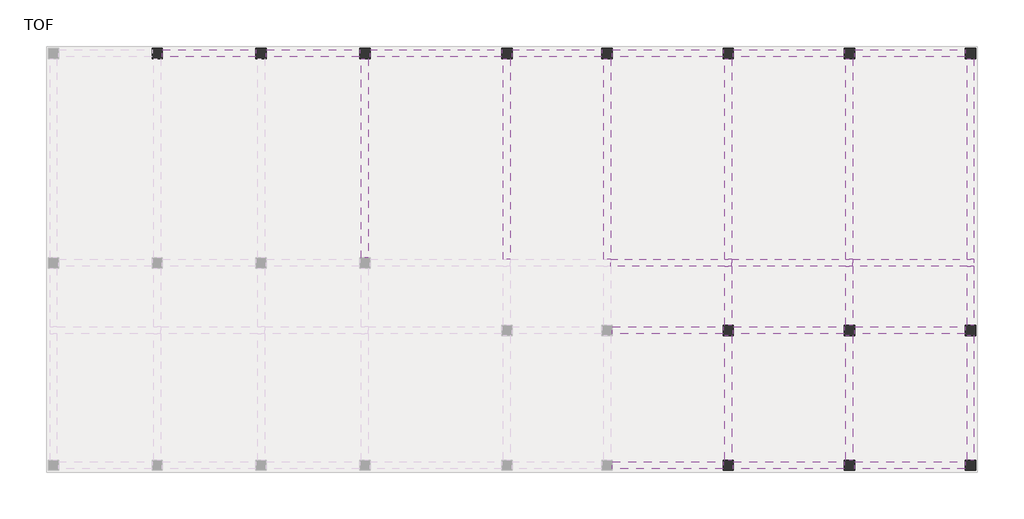
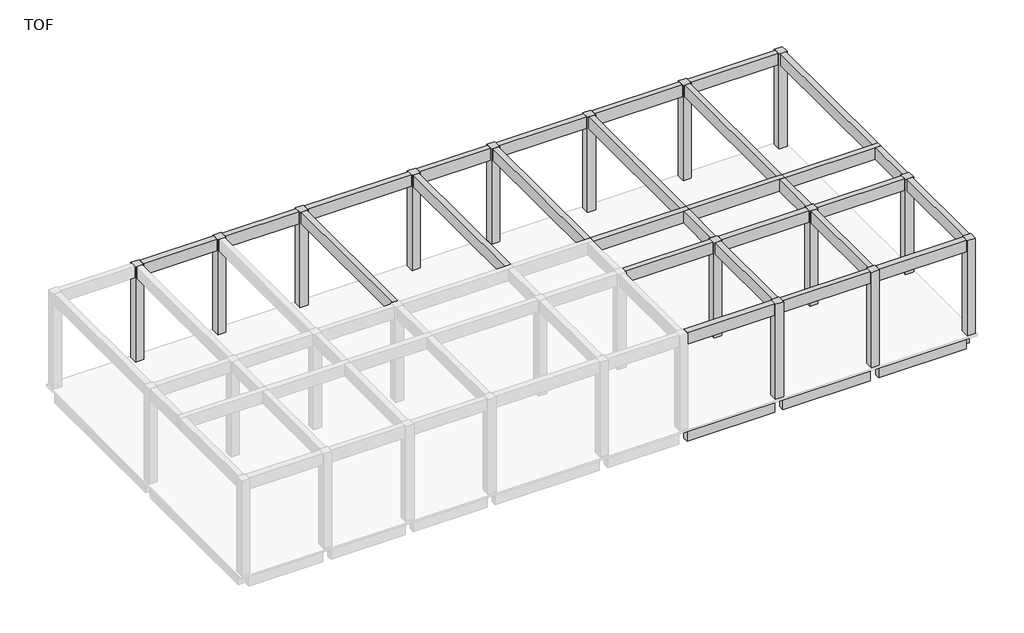
# One storey, part 2 of 2: 40 beams, 14 columns.
"""IFC4 building model written with IfcOpenShell, lengths in millimetres."""

from ifc_helpers import new_model, si_unit, frame, origin, place, context, project, spatial, polyline, outline, extrude, faceted_brep, element, save

model = new_model("IFC4")

# Units and contexts
model_context = context("Model", 3, world=origin())
ifc_project = project(units=[si_unit("LENGTHUNIT", "METRE", prefix="MILLI")], contexts=[model_context])

# Site, building, storey
site = spatial("IfcSite", under=ifc_project)
building = spatial("IfcBuilding", under=site)
storey = spatial("IfcBuildingStorey", under=building, Name="TOF", Elevation=150.0)

# Beams
placement = place(None, origin())
element("IfcBeam", 1, ObjectType="RC Beam_Rectangular : H_SB_ACB_B400xH900", at=placement, inside=storey, context=model_context, shape_type="SweptSolid", body=[
    extrude(outline(polyline([(52724.7, 24116.5208589), (53124.7, 24116.5208589), (53124.7, 18966.5208589), (52724.7, 18966.5208589), (52724.7, 24116.5208589)])), frame((0.0, 0.0, -900.0), z_axis=(0.0, 0.0, 1.0), x_axis=(1.0, 0.0, 0.0)), (0.0, 0.0, 1.0), 900.0),
    extrude(outline(polyline([(53124.7, 8716.5208589), (52724.7, 8716.5208589), (52724.7, 18366.5208589), (53124.7, 18366.5208589), (53124.7, 8716.5208589)])), frame((0.0, 0.0, -900.0), z_axis=(0.0, 0.0, 1.0), x_axis=(1.0, 0.0, 0.0)), (0.0, 0.0, 1.0), 900.0),
])
element("IfcBeam", 2, ObjectType="RC Beam_Rectangular : H_SB_ACB_B400xH900", at=placement, inside=storey, context=model_context, shape_type="SweptSolid", body=[
    extrude(outline(polyline([(52724.7, 8116.5208589), (53124.7, 8116.5208589), (53124.7, 916.5208589), (52724.7, 916.5208589), (52724.7, 8116.5208589)])), frame((0.0, 0.0, -900.0), z_axis=(0.0, 0.0, 1.0), x_axis=(1.0, 0.0, 0.0)), (0.0, 0.0, 1.0), 900.0),
])
element("IfcBeam", 3, ObjectType="RC Beam_Rectangular : H_SB_ACB_B400xH900", at=placement, inside=storey, context=model_context, shape_type="SweptSolid", body=[
    extrude(outline(polyline([(6224.7, 24216.5208589), (6224.7, 24616.5208589), (11624.7, 24616.5208589), (11624.7, 24216.5208589), (6224.7, 24216.5208589)])), frame((0.0, 0.0, -900.0), z_axis=(0.0, 0.0, 1.0), x_axis=(1.0, 0.0, 0.0)), (0.0, 0.0, 1.0), 900.0),
])
element("IfcBeam", 4, ObjectType="RC Beam_Rectangular : H_SB_ACB_B400xH900", at=placement, inside=storey, context=model_context, shape_type="SweptSolid", body=[
    extrude(outline(polyline([(12224.7, 24216.5208589), (12224.7, 24616.5208589), (17624.7, 24616.5208589), (17624.7, 24216.5208589), (12224.7, 24216.5208589)])), frame((0.0, 0.0, -900.0), z_axis=(0.0, 0.0, 1.0), x_axis=(1.0, 0.0, 0.0)), (0.0, 0.0, 1.0), 900.0),
])
element("IfcBeam", 5, ObjectType="RC Beam_Rectangular : H_SB_ACB_B400xH900", at=placement, inside=storey, context=model_context, shape_type="SweptSolid", body=[
    extrude(outline(polyline([(18224.7, 24216.5208589), (18224.7, 24616.5208589), (25824.7, 24616.5208589), (25824.7, 24216.5208589), (18224.7, 24216.5208589)])), frame((0.0, 0.0, -900.0), z_axis=(0.0, 0.0, 1.0), x_axis=(1.0, 0.0, 0.0)), (0.0, 0.0, 1.0), 900.0),
])
element("IfcBeam", 6, ObjectType="RC Beam_Rectangular : H_SB_ACB_B400xH900", at=placement, inside=storey, context=model_context, shape_type="SweptSolid", body=[
    extrude(outline(polyline([(26424.7, 24216.5208589), (26424.7, 24616.5208589), (31624.7, 24616.5208589), (31624.7, 24216.5208589), (26424.7, 24216.5208589)])), frame((0.0, 0.0, -900.0), z_axis=(0.0, 0.0, 1.0), x_axis=(1.0, 0.0, 0.0)), (0.0, 0.0, 1.0), 900.0),
])
element("IfcBeam", 7, ObjectType="RC Beam_Rectangular : H_SB_ACB_B400xH900", at=placement, inside=storey, context=model_context, shape_type="SweptSolid", body=[
    extrude(outline(polyline([(32224.7, 24216.5208589), (32224.7, 24616.5208589), (38624.7, 24616.5208589), (38624.7, 24216.5208589), (32224.7, 24216.5208589)])), frame((0.0, 0.0, -900.0), z_axis=(0.0, 0.0, 1.0), x_axis=(1.0, 0.0, 0.0)), (0.0, 0.0, 1.0), 900.0),
])
element("IfcBeam", 8, ObjectType="RC Beam_Rectangular : H_SB_ACB_B400xH900", at=placement, inside=storey, context=model_context, shape_type="SweptSolid", body=[
    extrude(outline(polyline([(39224.7, 24216.5208589), (39224.7, 24616.5208589), (45624.7, 24616.5208589), (45624.7, 24216.5208589), (39224.7, 24216.5208589)])), frame((0.0, 0.0, -900.0), z_axis=(0.0, 0.0, 1.0), x_axis=(1.0, 0.0, 0.0)), (0.0, 0.0, 1.0), 900.0),
])
element("IfcBeam", 9, ObjectType="RC Beam_Rectangular : H_SB_ACB_B400xH900", at=placement, inside=storey, context=model_context, shape_type="SweptSolid", body=[
    extrude(outline(polyline([(46224.7, 24216.5208589), (46224.7, 24616.5208589), (52624.7, 24616.5208589), (52624.7, 24216.5208589), (46224.7, 24216.5208589)])), frame((0.0, 0.0, -900.0), z_axis=(0.0, 0.0, 1.0), x_axis=(1.0, 0.0, 0.0)), (0.0, 0.0, 1.0), 900.0),
])
element("IfcBeam", 10, ObjectType="RC Beam_Rectangular : H_SB_ACB_B400xH900", at=placement, inside=storey, context=model_context, shape_type="SweptSolid", body=[
    extrude(outline(polyline([(32224.7, 416.5208589), (32224.7, 816.5208589), (38624.7, 816.5208589), (38624.7, 416.5208589), (32224.7, 416.5208589)])), frame((0.0, 0.0, -900.0), z_axis=(0.0, 0.0, 1.0), x_axis=(1.0, 0.0, 0.0)), (0.0, 0.0, 1.0), 900.0),
])
element("IfcBeam", 11, ObjectType="RC Beam_Rectangular : H_SB_ACB_B400xH900", at=placement, inside=storey, context=model_context, shape_type="SweptSolid", body=[
    extrude(outline(polyline([(39224.7, 416.5208589), (39224.7, 816.5208589), (45624.7, 816.5208589), (45624.7, 416.5208589), (39224.7, 416.5208589)])), frame((0.0, 0.0, -900.0), z_axis=(0.0, 0.0, 1.0), x_axis=(1.0, 0.0, 0.0)), (0.0, 0.0, 1.0), 900.0),
])
element("IfcBeam", 12, ObjectType="RC Beam_Rectangular : H_SB_ACB_B400xH900", at=placement, inside=storey, context=model_context, shape_type="SweptSolid", body=[
    extrude(outline(polyline([(46224.7, 416.5208589), (46224.7, 816.5208589), (52624.7, 816.5208589), (52624.7, 416.5208589), (46224.7, 416.5208589)])), frame((0.0, 0.0, -900.0), z_axis=(0.0, 0.0, 1.0), x_axis=(1.0, 0.0, 0.0)), (0.0, 0.0, 1.0), 900.0),
])
element("IfcBeam", 13, ObjectType="RC Beam_Rectangular : H_SB_ACB_B400xH900", at=placement, inside=storey, context=model_context, shape_type="Brep", body=[
    faceted_brep([(39124.7, 12116.5208589, 7500.0), (39124.7, 12516.5208589, 7500.0), (38724.7, 12516.5208589, 7500.0), (32124.7, 12516.5208589, 7500.0), (32124.7, 12116.5208589, 7500.0), (38724.7, 12116.5208589, 7500.0), (39124.7, 12116.5208589, 6600.0), (32124.7, 12116.5208589, 6600.0), (38724.7, 12116.5208589, 6600.0), (39124.7, 12516.5208589, 6600.0), (32124.7, 12516.5208589, 6600.0), (38724.7, 12516.5208589, 6600.0)], [[[0, 1, 2, 3, 4, 5]], [[6, 0, 5, 4, 7, 8]], [[9, 6, 8, 7, 10, 11]], [[1, 9, 11, 10, 3, 2]], [[1, 0, 6, 9]], [[4, 3, 10, 7]]]),
])
element("IfcBeam", 14, ObjectType="RC Beam_Rectangular : H_SB_ACB_B400xH900", at=placement, inside=storey, context=model_context, shape_type="Brep", body=[
    faceted_brep([(46124.7, 12116.5208589, 7500.0), (46124.7, 12516.5208589, 7500.0), (45724.7, 12516.5208589, 7500.0), (39124.7, 12516.5208589, 7500.0), (39124.7, 12116.5208589, 7500.0), (45724.7, 12116.5208589, 7500.0), (46124.7, 12116.5208589, 6600.0), (39124.7, 12116.5208589, 6600.0), (45724.7, 12116.5208589, 6600.0), (46124.7, 12516.5208589, 6600.0), (39124.7, 12516.5208589, 6600.0), (45724.7, 12516.5208589, 6600.0)], [[[0, 1, 2, 3, 4, 5]], [[6, 0, 5, 4, 7, 8]], [[9, 6, 8, 7, 10, 11]], [[1, 9, 11, 10, 3, 2]], [[1, 0, 6, 9]], [[4, 3, 10, 7]]]),
])
element("IfcBeam", 15, ObjectType="RC Beam_Rectangular : H_SB_ACB_B400xH900", at=placement, inside=storey, context=model_context, shape_type="Brep", body=[
    faceted_brep([(53124.7, 12116.5208589, 7500.0), (53124.7, 12516.5208589, 7500.0), (52724.7, 12516.5208589, 7500.0), (46124.7, 12516.5208589, 7500.0), (46124.7, 12116.5208589, 7500.0), (52724.7, 12116.5208589, 7500.0), (53124.7, 12116.5208589, 6600.0), (46124.7, 12116.5208589, 6600.0), (52724.7, 12116.5208589, 6600.0), (53124.7, 12516.5208589, 6600.0), (46124.7, 12516.5208589, 6600.0), (52724.7, 12516.5208589, 6600.0)], [[[0, 1, 2, 3, 4, 5]], [[6, 0, 5, 4, 7, 8]], [[9, 6, 8, 7, 10, 11]], [[1, 9, 11, 10, 3, 2]], [[1, 0, 6, 9]], [[4, 3, 10, 7]]]),
])
element("IfcBeam", 16, ObjectType="RC Beam_Rectangular : H_SB_ACB_B400xH900", at=placement, inside=storey, context=model_context, shape_type="SweptSolid", body=[
    extrude(outline(polyline([(6224.7, 24216.5208589), (6224.7, 24616.5208589), (11624.7, 24616.5208589), (11624.7, 24216.5208589), (6224.7, 24216.5208589)])), frame((0.0, 0.0, 6600.0), z_axis=(0.0, 0.0, 1.0), x_axis=(1.0, 0.0, 0.0)), (0.0, 0.0, 1.0), 900.0),
])
element("IfcBeam", 17, ObjectType="RC Beam_Rectangular : H_SB_ACB_B400xH900", at=placement, inside=storey, context=model_context, shape_type="SweptSolid", body=[
    extrude(outline(polyline([(12224.7, 24216.5208589), (12224.7, 24616.5208589), (17624.7, 24616.5208589), (17624.7, 24216.5208589), (12224.7, 24216.5208589)])), frame((0.0, 0.0, 6600.0), z_axis=(0.0, 0.0, 1.0), x_axis=(1.0, 0.0, 0.0)), (0.0, 0.0, 1.0), 900.0),
])
element("IfcBeam", 18, ObjectType="RC Beam_Rectangular : H_SB_ACB_B400xH900", at=placement, inside=storey, context=model_context, shape_type="SweptSolid", body=[
    extrude(outline(polyline([(18224.7, 24216.5208589), (18224.7, 24616.5208589), (25824.7, 24616.5208589), (25824.7, 24216.5208589), (18224.7, 24216.5208589)])), frame((0.0, 0.0, 6600.0), z_axis=(0.0, 0.0, 1.0), x_axis=(1.0, 0.0, 0.0)), (0.0, 0.0, 1.0), 900.0),
])
element("IfcBeam", 19, ObjectType="RC Beam_Rectangular : H_SB_ACB_B400xH900", at=placement, inside=storey, context=model_context, shape_type="SweptSolid", body=[
    extrude(outline(polyline([(26424.7, 24216.5208589), (26424.7, 24616.5208589), (31624.7, 24616.5208589), (31624.7, 24216.5208589), (26424.7, 24216.5208589)])), frame((0.0, 0.0, 6600.0), z_axis=(0.0, 0.0, 1.0), x_axis=(1.0, 0.0, 0.0)), (0.0, 0.0, 1.0), 900.0),
])
element("IfcBeam", 20, ObjectType="RC Beam_Rectangular : H_SB_ACB_B400xH900", at=placement, inside=storey, context=model_context, shape_type="SweptSolid", body=[
    extrude(outline(polyline([(32224.7, 24216.5208589), (32224.7, 24616.5208589), (38624.7, 24616.5208589), (38624.7, 24216.5208589), (32224.7, 24216.5208589)])), frame((0.0, 0.0, 6600.0), z_axis=(0.0, 0.0, 1.0), x_axis=(1.0, 0.0, 0.0)), (0.0, 0.0, 1.0), 900.0),
])
element("IfcBeam", 21, ObjectType="RC Beam_Rectangular : H_SB_ACB_B400xH900", at=placement, inside=storey, context=model_context, shape_type="SweptSolid", body=[
    extrude(outline(polyline([(39224.7, 24216.5208589), (39224.7, 24616.5208589), (45624.7, 24616.5208589), (45624.7, 24216.5208589), (39224.7, 24216.5208589)])), frame((0.0, 0.0, 6600.0), z_axis=(0.0, 0.0, 1.0), x_axis=(1.0, 0.0, 0.0)), (0.0, 0.0, 1.0), 900.0),
])
element("IfcBeam", 22, ObjectType="RC Beam_Rectangular : H_SB_ACB_B400xH900", at=placement, inside=storey, context=model_context, shape_type="SweptSolid", body=[
    extrude(outline(polyline([(46224.7, 24216.5208589), (46224.7, 24616.5208589), (52624.7, 24616.5208589), (52624.7, 24216.5208589), (46224.7, 24216.5208589)])), frame((0.0, 0.0, 6600.0), z_axis=(0.0, 0.0, 1.0), x_axis=(1.0, 0.0, 0.0)), (0.0, 0.0, 1.0), 900.0),
])
element("IfcBeam", 23, ObjectType="RC Beam_Rectangular : H_SB_ACB_B400xH900", at=placement, inside=storey, context=model_context, shape_type="SweptSolid", body=[
    extrude(outline(polyline([(32224.7, 8216.5208589), (32224.7, 8616.5208589), (38624.7, 8616.5208589), (38624.7, 8216.5208589), (32224.7, 8216.5208589)])), frame((0.0, 0.0, 6600.0), z_axis=(0.0, 0.0, 1.0), x_axis=(1.0, 0.0, 0.0)), (0.0, 0.0, 1.0), 900.0),
])
element("IfcBeam", 24, ObjectType="RC Beam_Rectangular : H_SB_ACB_B400xH900", at=placement, inside=storey, context=model_context, shape_type="SweptSolid", body=[
    extrude(outline(polyline([(39224.7, 8216.5208589), (39224.7, 8616.5208589), (45624.7, 8616.5208589), (45624.7, 8216.5208589), (39224.7, 8216.5208589)])), frame((0.0, 0.0, 6600.0), z_axis=(0.0, 0.0, 1.0), x_axis=(1.0, 0.0, 0.0)), (0.0, 0.0, 1.0), 900.0),
])
element("IfcBeam", 25, ObjectType="RC Beam_Rectangular : H_SB_ACB_B400xH900", at=placement, inside=storey, context=model_context, shape_type="SweptSolid", body=[
    extrude(outline(polyline([(46224.7, 8216.5208589), (46224.7, 8616.5208589), (52624.7, 8616.5208589), (52624.7, 8216.5208589), (46224.7, 8216.5208589)])), frame((0.0, 0.0, 6600.0), z_axis=(0.0, 0.0, 1.0), x_axis=(1.0, 0.0, 0.0)), (0.0, 0.0, 1.0), 900.0),
])
element("IfcBeam", 26, ObjectType="RC Beam_Rectangular : H_SB_ACB_B400xH900", at=placement, inside=storey, context=model_context, shape_type="SweptSolid", body=[
    extrude(outline(polyline([(32224.7, 416.5208589), (32224.7, 816.5208589), (38624.7, 816.5208589), (38624.7, 416.5208589), (32224.7, 416.5208589)])), frame((0.0, 0.0, 6600.0), z_axis=(0.0, 0.0, 1.0), x_axis=(1.0, 0.0, 0.0)), (0.0, 0.0, 1.0), 900.0),
])
element("IfcBeam", 27, ObjectType="RC Beam_Rectangular : H_SB_ACB_B400xH900", at=placement, inside=storey, context=model_context, shape_type="SweptSolid", body=[
    extrude(outline(polyline([(39224.7, 416.5208589), (39224.7, 816.5208589), (45624.7, 816.5208589), (45624.7, 416.5208589), (39224.7, 416.5208589)])), frame((0.0, 0.0, 6600.0), z_axis=(0.0, 0.0, 1.0), x_axis=(1.0, 0.0, 0.0)), (0.0, 0.0, 1.0), 900.0),
])
element("IfcBeam", 28, ObjectType="RC Beam_Rectangular : H_SB_ACB_B400xH900", at=placement, inside=storey, context=model_context, shape_type="SweptSolid", body=[
    extrude(outline(polyline([(46224.7, 416.5208589), (46224.7, 816.5208589), (52624.7, 816.5208589), (52624.7, 416.5208589), (46224.7, 416.5208589)])), frame((0.0, 0.0, 6600.0), z_axis=(0.0, 0.0, 1.0), x_axis=(1.0, 0.0, 0.0)), (0.0, 0.0, 1.0), 900.0),
])
element("IfcBeam", 29, ObjectType="RC Beam_Rectangular : H_SB_ACB_B400xH900", at=placement, inside=storey, context=model_context, shape_type="SweptSolid", body=[
    extrude(outline(polyline([(18124.7, 12616.5208589), (17724.7, 12616.5208589), (17724.7, 24116.5208589), (18124.7, 24116.5208589), (18124.7, 12616.5208589)])), frame((0.0, 0.0, 6600.0), z_axis=(0.0, 0.0, 1.0), x_axis=(1.0, 0.0, 0.0)), (0.0, 0.0, 1.0), 900.0),
])
element("IfcBeam", 30, ObjectType="RC Beam_Rectangular : H_SB_ACB_B400xH900", at=placement, inside=storey, context=model_context, shape_type="SweptSolid", body=[
    extrude(outline(polyline([(26324.7, 12516.5208589), (25924.7, 12516.5208589), (25924.7, 24116.5208589), (26324.7, 24116.5208589), (26324.7, 12516.5208589)])), frame((0.0, 0.0, 6600.0), z_axis=(0.0, 0.0, 1.0), x_axis=(1.0, 0.0, 0.0)), (0.0, 0.0, 1.0), 900.0),
])
element("IfcBeam", 31, ObjectType="RC Beam_Rectangular : H_SB_ACB_B400xH900", at=placement, inside=storey, context=model_context, shape_type="SweptSolid", body=[
    extrude(outline(polyline([(32124.7, 12516.5208589), (31724.7, 12516.5208589), (31724.7, 24116.5208589), (32124.7, 24116.5208589), (32124.7, 12516.5208589)])), frame((0.0, 0.0, 6600.0), z_axis=(0.0, 0.0, 1.0), x_axis=(1.0, 0.0, 0.0)), (0.0, 0.0, 1.0), 900.0),
])
element("IfcBeam", 32, ObjectType="RC Beam_Rectangular : H_SB_ACB_B400xH900", at=placement, inside=storey, context=model_context, shape_type="SweptSolid", body=[
    extrude(outline(polyline([(38724.7, 8116.5208589), (39124.7, 8116.5208589), (39124.7, 916.5208589), (38724.7, 916.5208589), (38724.7, 8116.5208589)])), frame((0.0, 0.0, 6600.0), z_axis=(0.0, 0.0, 1.0), x_axis=(1.0, 0.0, 0.0)), (0.0, 0.0, 1.0), 900.0),
])
element("IfcBeam", 33, ObjectType="RC Beam_Rectangular : H_SB_ACB_B400xH900", at=placement, inside=storey, context=model_context, shape_type="SweptSolid", body=[
    extrude(outline(polyline([(38724.7, 12116.5208589), (39124.7, 12116.5208589), (39124.7, 8716.5208589), (38724.7, 8716.5208589), (38724.7, 12116.5208589)])), frame((0.0, 0.0, 6600.0), z_axis=(0.0, 0.0, 1.0), x_axis=(1.0, 0.0, 0.0)), (0.0, 0.0, 1.0), 900.0),
])
element("IfcBeam", 34, ObjectType="RC Beam_Rectangular : H_SB_ACB_B400xH900", at=placement, inside=storey, context=model_context, shape_type="SweptSolid", body=[
    extrude(outline(polyline([(39124.7, 12516.5208589), (38724.7, 12516.5208589), (38724.7, 24116.5208589), (39124.7, 24116.5208589), (39124.7, 12516.5208589)])), frame((0.0, 0.0, 6600.0), z_axis=(0.0, 0.0, 1.0), x_axis=(1.0, 0.0, 0.0)), (0.0, 0.0, 1.0), 900.0),
])
element("IfcBeam", 35, ObjectType="RC Beam_Rectangular : H_SB_ACB_B400xH900", at=placement, inside=storey, context=model_context, shape_type="SweptSolid", body=[
    extrude(outline(polyline([(45724.7, 8116.5208589), (46124.7, 8116.5208589), (46124.7, 916.5208589), (45724.7, 916.5208589), (45724.7, 8116.5208589)])), frame((0.0, 0.0, 6600.0), z_axis=(0.0, 0.0, 1.0), x_axis=(1.0, 0.0, 0.0)), (0.0, 0.0, 1.0), 900.0),
])
element("IfcBeam", 36, ObjectType="RC Beam_Rectangular : H_SB_ACB_B400xH900", at=placement, inside=storey, context=model_context, shape_type="SweptSolid", body=[
    extrude(outline(polyline([(45724.7, 12116.5208589), (46124.7, 12116.5208589), (46124.7, 8716.5208589), (45724.7, 8716.5208589), (45724.7, 12116.5208589)])), frame((0.0, 0.0, 6600.0), z_axis=(0.0, 0.0, 1.0), x_axis=(1.0, 0.0, 0.0)), (0.0, 0.0, 1.0), 900.0),
])
element("IfcBeam", 37, ObjectType="RC Beam_Rectangular : H_SB_ACB_B400xH900", at=placement, inside=storey, context=model_context, shape_type="SweptSolid", body=[
    extrude(outline(polyline([(46124.7, 12516.5208589), (45724.7, 12516.5208589), (45724.7, 24116.5208589), (46124.7, 24116.5208589), (46124.7, 12516.5208589)])), frame((0.0, 0.0, 6600.0), z_axis=(0.0, 0.0, 1.0), x_axis=(1.0, 0.0, 0.0)), (0.0, 0.0, 1.0), 900.0),
])
element("IfcBeam", 38, ObjectType="RC Beam_Rectangular : H_SB_ACB_B400xH900", at=placement, inside=storey, context=model_context, shape_type="SweptSolid", body=[
    extrude(outline(polyline([(52724.7, 8116.5208589), (53124.7, 8116.5208589), (53124.7, 916.5208589), (52724.7, 916.5208589), (52724.7, 8116.5208589)])), frame((0.0, 0.0, 6600.0), z_axis=(0.0, 0.0, 1.0), x_axis=(1.0, 0.0, 0.0)), (0.0, 0.0, 1.0), 900.0),
])
element("IfcBeam", 39, ObjectType="RC Beam_Rectangular : H_SB_ACB_B400xH900", at=placement, inside=storey, context=model_context, shape_type="SweptSolid", body=[
    extrude(outline(polyline([(52724.7, 12116.5208589), (53124.7, 12116.5208589), (53124.7, 8716.5208589), (52724.7, 8716.5208589), (52724.7, 12116.5208589)])), frame((0.0, 0.0, 6600.0), z_axis=(0.0, 0.0, 1.0), x_axis=(1.0, 0.0, 0.0)), (0.0, 0.0, 1.0), 900.0),
])
element("IfcBeam", 40, ObjectType="RC Beam_Rectangular : H_SB_ACB_B400xH900", at=placement, inside=storey, context=model_context, shape_type="SweptSolid", body=[
    extrude(outline(polyline([(52724.7, 24116.5208589), (53124.7, 24116.5208589), (53124.7, 12516.5208589), (52724.7, 12516.5208589), (52724.7, 24116.5208589)])), frame((0.0, 0.0, 6600.0), z_axis=(0.0, 0.0, 1.0), x_axis=(1.0, 0.0, 0.0)), (0.0, 0.0, 1.0), 900.0),
])

# Columns
element("IfcColumn", 41, ObjectType="RC_Column_Rectangular : H_SC_ACC_W600xL600", at=placement, inside=storey, context=model_context, shape_type="Brep", body=[
    faceted_brep([(6224.7, 24716.5208589, 7500.0), (6224.7, 24616.5208589, 7500.0), (6224.7, 24216.5208589, 7500.0), (6224.7, 24116.5208589, 7500.0), (6224.7, 24116.5208589, 150.0), (6224.7, 24716.5208589, 150.0), (6124.7, 24116.5208589, 7500.0), (5724.7, 24116.5208589, 7500.0), (5624.7, 24116.5208589, 7500.0), (5624.7, 24116.5208589, 150.0), (5624.7, 24216.5208589, 7500.0), (5624.7, 24616.5208589, 7500.0), (5624.7, 24716.5208589, 7500.0), (5624.7, 24716.5208589, 150.0)], [[[0, 1, 2, 3, 4, 5]], [[3, 6, 7, 8, 9, 4]], [[8, 10, 11, 12, 13, 9]], [[12, 0, 5, 13]], [[3, 2, 1, 0, 12, 11, 10, 8, 7, 6]], [[5, 4, 9, 13]]]),
])
element("IfcColumn", 42, ObjectType="RC_Column_Rectangular : H_SC_ACC_W600xL600", at=placement, inside=storey, context=model_context, shape_type="Brep", body=[
    faceted_brep([(12224.7, 24716.5208589, 7500.0), (12224.7, 24616.5208589, 7500.0), (12224.7, 24216.5208589, 7500.0), (12224.7, 24116.5208589, 7500.0), (12224.7, 24116.5208589, 150.0), (12224.7, 24716.5208589, 150.0), (12124.7, 24116.5208589, 7500.0), (11724.7, 24116.5208589, 7500.0), (11624.7, 24116.5208589, 7500.0), (11624.7, 24116.5208589, 150.0), (11624.7, 24216.5208589, 7500.0), (11624.7, 24616.5208589, 7500.0), (11624.7, 24716.5208589, 7500.0), (11624.7, 24716.5208589, 150.0)], [[[0, 1, 2, 3, 4, 5]], [[3, 6, 7, 8, 9, 4]], [[8, 10, 11, 12, 13, 9]], [[12, 0, 5, 13]], [[3, 2, 1, 0, 12, 11, 10, 8, 7, 6]], [[5, 4, 9, 13]]]),
])
element("IfcColumn", 43, ObjectType="RC_Column_Rectangular : H_SC_ACC_W600xL600", at=placement, inside=storey, context=model_context, shape_type="Brep", body=[
    faceted_brep([(18224.7, 24716.5208589, 7500.0), (18224.7, 24616.5208589, 7500.0), (18224.7, 24216.5208589, 7500.0), (18224.7, 24116.5208589, 7500.0), (18224.7, 24116.5208589, 150.0), (18224.7, 24716.5208589, 150.0), (18124.7, 24116.5208589, 7500.0), (17724.7, 24116.5208589, 7500.0), (17624.7, 24116.5208589, 7500.0), (17624.7, 24116.5208589, 150.0), (17624.7, 24216.5208589, 7500.0), (17624.7, 24616.5208589, 7500.0), (17624.7, 24716.5208589, 7500.0), (17624.7, 24716.5208589, 150.0)], [[[0, 1, 2, 3, 4, 5]], [[3, 6, 7, 8, 9, 4]], [[8, 10, 11, 12, 13, 9]], [[12, 0, 5, 13]], [[3, 2, 1, 0, 12, 11, 10, 8, 7, 6]], [[5, 4, 9, 13]]]),
])
element("IfcColumn", 44, ObjectType="RC_Column_Rectangular : H_SC_ACC_W600xL600", at=placement, inside=storey, context=model_context, shape_type="Brep", body=[
    faceted_brep([(26424.7, 24716.5208589, 7500.0), (26424.7, 24616.5208589, 7500.0), (26424.7, 24216.5208589, 7500.0), (26424.7, 24116.5208589, 7500.0), (26424.7, 24116.5208589, 150.0), (26424.7, 24716.5208589, 150.0), (26324.7, 24116.5208589, 7500.0), (25924.7, 24116.5208589, 7500.0), (25824.7, 24116.5208589, 7500.0), (25824.7, 24116.5208589, 150.0), (25824.7, 24216.5208589, 7500.0), (25824.7, 24616.5208589, 7500.0), (25824.7, 24716.5208589, 7500.0), (25824.7, 24716.5208589, 150.0)], [[[0, 1, 2, 3, 4, 5]], [[3, 6, 7, 8, 9, 4]], [[8, 10, 11, 12, 13, 9]], [[12, 0, 5, 13]], [[3, 2, 1, 0, 12, 11, 10, 8, 7, 6]], [[5, 4, 9, 13]]]),
])
element("IfcColumn", 45, ObjectType="RC_Column_Rectangular : H_SC_ACC_W600xL600", at=placement, inside=storey, context=model_context, shape_type="Brep", body=[
    faceted_brep([(32224.7, 24716.5208589, 7500.0), (32224.7, 24616.5208589, 7500.0), (32224.7, 24216.5208589, 7500.0), (32224.7, 24116.5208589, 7500.0), (32224.7, 24116.5208589, 150.0), (32224.7, 24716.5208589, 150.0), (32124.7, 24116.5208589, 7500.0), (31724.7, 24116.5208589, 7500.0), (31624.7, 24116.5208589, 7500.0), (31624.7, 24116.5208589, 150.0), (31624.7, 24216.5208589, 7500.0), (31624.7, 24616.5208589, 7500.0), (31624.7, 24716.5208589, 7500.0), (31624.7, 24716.5208589, 150.0)], [[[0, 1, 2, 3, 4, 5]], [[3, 6, 7, 8, 9, 4]], [[8, 10, 11, 12, 13, 9]], [[12, 0, 5, 13]], [[3, 2, 1, 0, 12, 11, 10, 8, 7, 6]], [[5, 4, 9, 13]]]),
])
element("IfcColumn", 46, ObjectType="RC_Column_Rectangular : H_SC_ACC_W600xL600", at=placement, inside=storey, context=model_context, shape_type="Brep", body=[
    faceted_brep([(39224.7, 24716.5208589, 7500.0), (39224.7, 24616.5208589, 7500.0), (39224.7, 24216.5208589, 7500.0), (39224.7, 24116.5208589, 7500.0), (39224.7, 24116.5208589, 150.0), (39224.7, 24716.5208589, 150.0), (39124.7, 24116.5208589, 7500.0), (38724.7, 24116.5208589, 7500.0), (38624.7, 24116.5208589, 7500.0), (38624.7, 24116.5208589, 150.0), (38624.7, 24216.5208589, 7500.0), (38624.7, 24616.5208589, 7500.0), (38624.7, 24716.5208589, 7500.0), (38624.7, 24716.5208589, 150.0)], [[[0, 1, 2, 3, 4, 5]], [[3, 6, 7, 8, 9, 4]], [[8, 10, 11, 12, 13, 9]], [[12, 0, 5, 13]], [[3, 2, 1, 0, 12, 11, 10, 8, 7, 6]], [[5, 4, 9, 13]]]),
])
element("IfcColumn", 47, ObjectType="RC_Column_Rectangular : H_SC_ACC_W600xL600", at=placement, inside=storey, context=model_context, shape_type="Brep", body=[
    faceted_brep([(46224.7, 24716.5208589, 7500.0), (46224.7, 24616.5208589, 7500.0), (46224.7, 24216.5208589, 7500.0), (46224.7, 24116.5208589, 7500.0), (46224.7, 24116.5208589, 150.0), (46224.7, 24716.5208589, 150.0), (46124.7, 24116.5208589, 7500.0), (45724.7, 24116.5208589, 7500.0), (45624.7, 24116.5208589, 7500.0), (45624.7, 24116.5208589, 150.0), (45624.7, 24216.5208589, 7500.0), (45624.7, 24616.5208589, 7500.0), (45624.7, 24716.5208589, 7500.0), (45624.7, 24716.5208589, 150.0)], [[[0, 1, 2, 3, 4, 5]], [[3, 6, 7, 8, 9, 4]], [[8, 10, 11, 12, 13, 9]], [[12, 0, 5, 13]], [[3, 2, 1, 0, 12, 11, 10, 8, 7, 6]], [[5, 4, 9, 13]]]),
])
element("IfcColumn", 48, ObjectType="RC_Column_Rectangular : H_SC_ACC_W600xL600", at=placement, inside=storey, context=model_context, shape_type="Brep", body=[
    faceted_brep([(53224.7, 24716.5208589, 7500.0), (53224.7, 24116.5208589, 7500.0), (53224.7, 24116.5208589, 150.0), (53224.7, 24716.5208589, 150.0), (53124.7, 24116.5208589, 7500.0), (52724.7, 24116.5208589, 7500.0), (52624.7, 24116.5208589, 7500.0), (52624.7, 24116.5208589, 150.0), (52624.7, 24216.5208589, 7500.0), (52624.7, 24616.5208589, 7500.0), (52624.7, 24716.5208589, 7500.0), (52624.7, 24716.5208589, 150.0)], [[[0, 1, 2, 3]], [[1, 4, 5, 6, 7, 2]], [[6, 8, 9, 10, 11, 7]], [[10, 0, 3, 11]], [[1, 0, 10, 9, 8, 6, 5, 4]], [[3, 2, 7, 11]]]),
])
element("IfcColumn", 49, ObjectType="RC_Column_Rectangular : H_SC_ACC_W600xL600", at=placement, inside=storey, context=model_context, shape_type="Brep", body=[
    faceted_brep([(39224.7, 8716.5208589, 7500.0), (39224.7, 8616.5208589, 7500.0), (39224.7, 8216.5208589, 7500.0), (39224.7, 8116.5208589, 7500.0), (39224.7, 8116.5208589, 150.0), (39224.7, 8716.5208589, 150.0), (39124.7, 8116.5208589, 7500.0), (38724.7, 8116.5208589, 7500.0), (38624.7, 8116.5208589, 7500.0), (38624.7, 8116.5208589, 150.0), (38624.7, 8216.5208589, 7500.0), (38624.7, 8616.5208589, 7500.0), (38624.7, 8716.5208589, 7500.0), (38624.7, 8716.5208589, 150.0), (38724.7, 8716.5208589, 7500.0), (39124.7, 8716.5208589, 7500.0)], [[[0, 1, 2, 3, 4, 5]], [[3, 6, 7, 8, 9, 4]], [[8, 10, 11, 12, 13, 9]], [[12, 14, 15, 0, 5, 13]], [[3, 2, 1, 0, 15, 14, 12, 11, 10, 8, 7, 6]], [[5, 4, 9, 13]]]),
])
element("IfcColumn", 50, ObjectType="RC_Column_Rectangular : H_SC_ACC_W600xL600", at=placement, inside=storey, context=model_context, shape_type="Brep", body=[
    faceted_brep([(46224.7, 8716.5208589, 7500.0), (46224.7, 8616.5208589, 7500.0), (46224.7, 8216.5208589, 7500.0), (46224.7, 8116.5208589, 7500.0), (46224.7, 8116.5208589, 150.0), (46224.7, 8716.5208589, 150.0), (46124.7, 8116.5208589, 7500.0), (45724.7, 8116.5208589, 7500.0), (45624.7, 8116.5208589, 7500.0), (45624.7, 8116.5208589, 150.0), (45624.7, 8216.5208589, 7500.0), (45624.7, 8616.5208589, 7500.0), (45624.7, 8716.5208589, 7500.0), (45624.7, 8716.5208589, 150.0), (45724.7, 8716.5208589, 7500.0), (46124.7, 8716.5208589, 7500.0)], [[[0, 1, 2, 3, 4, 5]], [[3, 6, 7, 8, 9, 4]], [[8, 10, 11, 12, 13, 9]], [[12, 14, 15, 0, 5, 13]], [[3, 2, 1, 0, 15, 14, 12, 11, 10, 8, 7, 6]], [[5, 4, 9, 13]]]),
])
element("IfcColumn", 51, ObjectType="RC_Column_Rectangular : H_SC_ACC_W600xL600", at=placement, inside=storey, context=model_context, shape_type="Brep", body=[
    faceted_brep([(53224.7, 8716.5208589, 7500.0), (53224.7, 8116.5208589, 7500.0), (53224.7, 8116.5208589, 150.0), (53224.7, 8716.5208589, 150.0), (53124.7, 8116.5208589, 7500.0), (52724.7, 8116.5208589, 7500.0), (52624.7, 8116.5208589, 7500.0), (52624.7, 8116.5208589, 150.0), (52624.7, 8216.5208589, 7500.0), (52624.7, 8616.5208589, 7500.0), (52624.7, 8716.5208589, 7500.0), (52624.7, 8716.5208589, 150.0), (52724.7, 8716.5208589, 7500.0), (53124.7, 8716.5208589, 7500.0)], [[[0, 1, 2, 3]], [[1, 4, 5, 6, 7, 2]], [[6, 8, 9, 10, 11, 7]], [[10, 12, 13, 0, 3, 11]], [[1, 0, 13, 12, 10, 9, 8, 6, 5, 4]], [[3, 2, 7, 11]]]),
])
element("IfcColumn", 52, ObjectType="RC_Column_Rectangular : H_SC_ACC_W600xL600", at=placement, inside=storey, context=model_context, shape_type="Brep", body=[
    faceted_brep([(39224.7, 916.5208589, 7500.0), (39224.7, 816.5208589, 7500.0), (39224.7, 416.5208589, 7500.0), (39224.7, 316.5208589, 7500.0), (39224.7, 316.5208589, 150.0), (39224.7, 916.5208589, 150.0), (38624.7, 316.5208589, 7500.0), (38624.7, 316.5208589, 150.0), (38624.7, 416.5208589, 7500.0), (38624.7, 816.5208589, 7500.0), (38624.7, 916.5208589, 7500.0), (38624.7, 916.5208589, 150.0), (38724.7, 916.5208589, 7500.0), (39124.7, 916.5208589, 7500.0)], [[[0, 1, 2, 3, 4, 5]], [[3, 6, 7, 4]], [[6, 8, 9, 10, 11, 7]], [[10, 12, 13, 0, 5, 11]], [[3, 2, 1, 0, 13, 12, 10, 9, 8, 6]], [[5, 4, 7, 11]]]),
])
element("IfcColumn", 53, ObjectType="RC_Column_Rectangular : H_SC_ACC_W600xL600", at=placement, inside=storey, context=model_context, shape_type="Brep", body=[
    faceted_brep([(46224.7, 916.5208589, 7500.0), (46224.7, 816.5208589, 7500.0), (46224.7, 416.5208589, 7500.0), (46224.7, 316.5208589, 7500.0), (46224.7, 316.5208589, 150.0), (46224.7, 916.5208589, 150.0), (45624.7, 316.5208589, 7500.0), (45624.7, 316.5208589, 150.0), (45624.7, 416.5208589, 7500.0), (45624.7, 816.5208589, 7500.0), (45624.7, 916.5208589, 7500.0), (45624.7, 916.5208589, 150.0), (45724.7, 916.5208589, 7500.0), (46124.7, 916.5208589, 7500.0)], [[[0, 1, 2, 3, 4, 5]], [[3, 6, 7, 4]], [[6, 8, 9, 10, 11, 7]], [[10, 12, 13, 0, 5, 11]], [[3, 2, 1, 0, 13, 12, 10, 9, 8, 6]], [[5, 4, 7, 11]]]),
])
element("IfcColumn", 54, ObjectType="RC_Column_Rectangular : H_SC_ACC_W600xL600", at=placement, inside=storey, context=model_context, shape_type="Brep", body=[
    faceted_brep([(53224.7, 916.5208589, 7500.0), (53224.7, 316.5208589, 7500.0), (53224.7, 316.5208589, 150.0), (53224.7, 916.5208589, 150.0), (52624.7, 316.5208589, 7500.0), (52624.7, 316.5208589, 150.0), (52624.7, 416.5208589, 7500.0), (52624.7, 816.5208589, 7500.0), (52624.7, 916.5208589, 7500.0), (52624.7, 916.5208589, 150.0), (52724.7, 916.5208589, 7500.0), (53124.7, 916.5208589, 7500.0)], [[[0, 1, 2, 3]], [[1, 4, 5, 2]], [[4, 6, 7, 8, 9, 5]], [[8, 10, 11, 0, 3, 9]], [[1, 0, 11, 10, 8, 7, 6, 4]], [[3, 2, 5, 9]]]),
])

save(model, "model.ifc")

# Revit data of these elements
# Type "RC Beam_Rectangular : H_SB_ACB_B400xH900"
#   중앙부 하부근 = ""
#   중앙부 상부근 = ""
#   중앙부 보조근 = ""
#   중앙부 늑근 = ""
#   외단부 하부근 = ""
#   외단부 상부근 = ""
#   외단부 보조근 = ""
#   외단부 늑근 = ""
#   부호 = "TG3"
#   내단부 하부근 = ""
#   내단부 상부근 = ""
#   내단부 보조근 = ""
#   내단부 늑근 = ""
#   ALL 하부근 = "3-D20"
#   ALL 상부근 = "3-D20"
#   ALL 보조근 = ""
#   ALL 늑근 = "2-D10 @120"
#   Width = 400.000 mm
#   Height = 900.000 mm
#   Length [instance default] = 1524.000 mm
#   b = 400.000 mm
#   h = 900.000 mm
#   hec_material3 [instance default] = none
#   hec_material2 [instance default] = none
#   hec_material1 [instance default] = none
#   Structural Material [instance default] = none
#   Assembly Code = ""
# Type "RC_Column_Rectangular : H_SC_ACC_W600xL600"
#   Width = 600.000 mm
#   Length = 600.000 mm
#   hec_material3 [instance default] = none
#   hec_material2 [instance default] = none
#   hec_material1 [instance default] = none
#   Structural Material [instance default] = none
#   Description = (empty or 0)
# Elements 1, 2, 3, 4, 5, 6, 7, 8, 9, 10, 11, 12, 13, 14, 15, 16, 17, 18, 19, 20, 21, 22, 23, 24, 25, 26, 27, 28, 29, 30, 31, 32, 33, 34, 35, 36, 37, 38, 39, 40 (IfcBeam, "RC Beam_Rectangular : H_SB_ACB_B400xH900")
#   hec_material3 = none
#   hec_material2 = none
#   hec_material1 = none
#   Structural Material = none
#   Phase Created = New Construction
# Elements 41, 42, 43, 44, 45, 46, 47, 48, 49, 50, 51, 52, 53, 54 (IfcColumn, "RC_Column_Rectangular : H_SC_ACC_W600xL600")
#   Comments = ""
#   hec_material3 = none
#   hec_material2 = none
#   hec_material1 = none
#   Structural Material = none
#   Phase Created = New Construction
